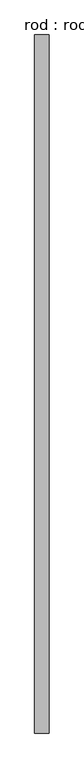
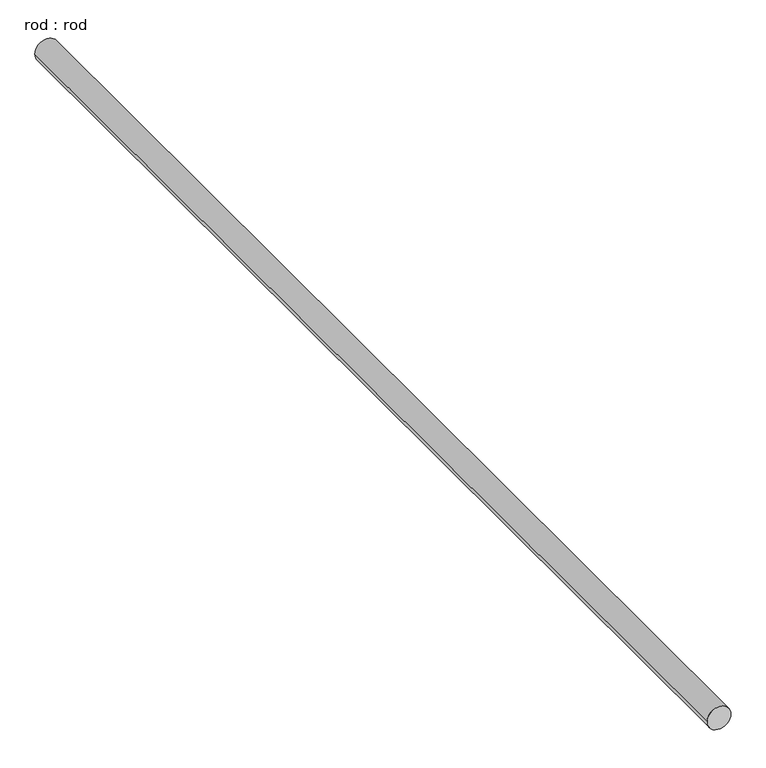
"""IFC4 building model written with IfcOpenShell, lengths in millimetres: proxy geometry, rod : rod."""

import ifcopenshell
import ifcopenshell.guid

model = None  # the IFC model being written
_history = None  # IfcOwnerHistory: only IFC2X3 demands one
_inside = {}  # id of a spatial element -> (the spatial element, [elements in it])
_under = {}  # id of a project, library or spatial element -> (it, [spatial elements below it])
_declared = {}  # id of a project -> (the project, [libraries it declares])
_typed = {}  # id of a type object -> (the type object, [elements of that type])
_made_of = {}  # id of a material, layer set ... -> (it, [elements and type objects made of it])


def new_model(schema):
    """Start an empty IFC model of exactly this schema.

    Asked for "IFC4X3", IfcOpenShell would pick the latest addendum, in which some entities
    have other attributes; the version numbers below select the first issue.
    IFC2X3 requires an IfcOwnerHistory on every rooted entity: one is made here for all.
    """
    global model, _history
    if schema == "IFC4X3":
        model = ifcopenshell.file(schema_version=(4, 3, 0, 0))
    else:
        model = ifcopenshell.file(schema=schema)
    _inside.clear()
    _under.clear()
    _declared.clear()
    _typed.clear()
    _made_of.clear()
    _history = None
    if model.schema == "IFC2X3":
        org = make("IfcOrganization", Name="unknown")
        user = make(
            "IfcPersonAndOrganization",
            ThePerson=make("IfcPerson", FamilyName="unknown"),
            TheOrganization=org,
        )
        app = make(
            "IfcApplication",
            ApplicationDeveloper=org,
            Version="unknown",
            ApplicationFullName="unknown",
            ApplicationIdentifier="unknown",
        )
        _history = make(
            "IfcOwnerHistory",
            OwningUser=user,
            OwningApplication=app,
            ChangeAction="ADDED",
            CreationDate=0,
        )
    return model


def make(cls, **values):
    """One entity of the class cls with the attributes given. An attribute that is None is left unset."""
    return model.create_entity(
        cls, **{name: value for name, value in values.items() if value is not None}
    )


def rooted(cls, **values):
    """An entity with a GlobalId (a new one), such as an element, a storey or a relation."""
    return make(cls, GlobalId=ifcopenshell.guid.new(), OwnerHistory=_history, **values)


def si_unit(unit_type, name, prefix=None):
    """IfcSIUnit, for example si_unit("LENGTHUNIT", "METRE", prefix="MILLI")."""
    return make("IfcSIUnit", UnitType=unit_type, Prefix=prefix, Name=name)


def assignment(units):
    """IfcUnitAssignment: the units of a project."""
    return None if units is None else make("IfcUnitAssignment", Units=units)


def point(xyz):
    """IfcCartesianPoint."""
    return None if xyz is None else make("IfcCartesianPoint", Coordinates=xyz)


def direction(xyz):
    """IfcDirection."""
    return None if xyz is None else make("IfcDirection", DirectionRatios=xyz)


def frame(location, z_axis=None, x_axis=None):
    """IfcAxis2Placement3D, a coordinate frame: its origin and axes. An axis left out is left unset."""
    return make(
        "IfcAxis2Placement3D",
        Location=point(location),
        Axis=direction(z_axis),
        RefDirection=direction(x_axis),
    )


def frame_2d(location, x_axis=None):
    """IfcAxis2Placement2D, a coordinate frame in the plane: its origin and x axis."""
    return make(
        "IfcAxis2Placement2D", Location=point(location), RefDirection=direction(x_axis)
    )


def origin():
    """The frame at (0, 0, 0) with its axes left unset."""
    return frame((0.0, 0.0, 0.0))


def place(relative_to, where):
    """IfcLocalPlacement: puts the frame where relative to a parent placement (None: the world)."""
    return make(
        "IfcLocalPlacement", PlacementRelTo=relative_to, RelativePlacement=where
    )


def context(
    kind, dimensions, precision=None, world=None, true_north=None, identifier=None
):
    """IfcGeometricRepresentationContext, for example the 3D "Model" context."""
    return make(
        "IfcGeometricRepresentationContext",
        ContextIdentifier=identifier,
        ContextType=kind,
        CoordinateSpaceDimension=dimensions,
        Precision=precision,
        WorldCoordinateSystem=world,
        TrueNorth=true_north,
    )


def project(units=None, contexts=None):
    """IfcProject with its units and contexts."""
    return rooted(
        "IfcProject",
        Name="project",
        RepresentationContexts=contexts,
        UnitsInContext=assignment(units),
    )


def spatial(cls, under=None, at=None, **own):
    """A site, building, storey or space (cls), placed at a placement, below another one or the project."""
    s = rooted(cls, ObjectPlacement=at, **own)
    if under is not None:
        _under.setdefault(under.id(), (under, []))[1].append(s)
    return s


def circle_curve(where, radius):
    """IfcCircle in the frame where."""
    return make("IfcCircle", Position=where, Radius=radius)


def trimmed(basis, trim1, trim2, sense, master):
    """IfcTrimmedCurve: the piece of a basis curve between two trims."""
    return make(
        "IfcTrimmedCurve",
        BasisCurve=basis,
        Trim1=trim1,
        Trim2=trim2,
        SenseAgreement=sense,
        MasterRepresentation=master,
    )


def segment(curve, same_sense, transition):
    """IfcCompositeCurveSegment."""
    return make(
        "IfcCompositeCurveSegment",
        Transition=transition,
        SameSense=same_sense,
        ParentCurve=curve,
    )


def composite_curve(segments, self_intersect=None):
    """IfcCompositeCurve: segments joined end to end."""
    return make("IfcCompositeCurve", Segments=segments, SelfIntersect=self_intersect)


def outline(outer, holes=None, kind="AREA"):
    """IfcArbitraryClosedProfileDef: a profile drawn as a closed curve; with holes, ...WithVoids."""
    if holes is None:
        return make("IfcArbitraryClosedProfileDef", ProfileType=kind, OuterCurve=outer)
    return make(
        "IfcArbitraryProfileDefWithVoids",
        ProfileType=kind,
        OuterCurve=outer,
        InnerCurves=holes,
    )


def extrude(swept, where, along, depth):
    """IfcExtrudedAreaSolid: the profile swept, set in the frame where, extruded along a direction by depth."""
    return make(
        "IfcExtrudedAreaSolid",
        SweptArea=swept,
        Position=where,
        ExtrudedDirection=direction(along),
        Depth=depth,
    )


def shape(context_of_items, identifier, shape_type, items):
    """IfcShapeRepresentation: the items that make up one representation, for example the "Body"."""
    return make(
        "IfcShapeRepresentation",
        ContextOfItems=context_of_items,
        RepresentationIdentifier=identifier,
        RepresentationType=shape_type,
        Items=items,
    )


def source(mapping_origin, context_of_items, identifier, shape_type, items):
    """IfcRepresentationMap: a shape defined once, which mapped items show again and again."""
    return make(
        "IfcRepresentationMap",
        MappingOrigin=mapping_origin,
        MappedRepresentation=shape(context_of_items, identifier, shape_type, items),
    )


def transform(
    local_origin,
    x_axis=None,
    y_axis=None,
    z_axis=None,
    scale=None,
    scale2=None,
    scale3=None,
    uniform=True,
):
    """IfcCartesianTransformationOperator3D, or its non-uniform kind. x_axis, y_axis, z_axis: its Axis1, 2, 3."""
    if uniform:
        return make(
            "IfcCartesianTransformationOperator3D",
            Axis1=direction(x_axis),
            Axis2=direction(y_axis),
            LocalOrigin=point(local_origin),
            Scale=scale,
            Axis3=direction(z_axis),
        )
    return make(
        "IfcCartesianTransformationOperator3DnonUniform",
        Axis1=direction(x_axis),
        Axis2=direction(y_axis),
        LocalOrigin=point(local_origin),
        Scale=scale,
        Axis3=direction(z_axis),
        Scale2=scale2,
        Scale3=scale3,
    )


def mapped(mapping_source, mapping_target):
    """IfcMappedItem: shows the shape of a source again, moved by a transform."""
    return make(
        "IfcMappedItem", MappingSource=mapping_source, MappingTarget=mapping_target
    )


def made_of(thing, what):
    """Note that an element or type object is made of a material, layer set ...; save() writes the relation."""
    if what is not None:
        _made_of.setdefault(what.id(), (what, []))[1].append(thing)
    return thing


def element(
    cls,
    number,
    at=None,
    inside=None,
    cuts=None,
    type_object=None,
    material=None,
    context=None,
    identifier="Body",
    shape_type=None,
    held_by="IfcProductDefinitionShape",
    body=None,
    shapes=None,
    **own,
):
    """One element of the class cls, such as IfcWall. Its Tag is "e" and its number.

    at: its placement. inside: the storey or other place that contains it. cuts: it is an
    opening in that element (IfcRelVoidsElement). A single representation is given by context,
    identifier, shape_type and body (its items); several are given by shapes. held_by: the class
    of the entity that holds the representations. save() writes the other relations.
    """
    e = rooted(cls, Tag="e%d" % number, ObjectPlacement=at, **own)
    if body is not None:
        shapes = [shape(context, identifier, shape_type, body)]
    if shapes is not None:
        e.Representation = make(held_by, Representations=shapes)
    if inside is not None:
        _inside.setdefault(inside.id(), (inside, []))[1].append(e)
    if cuts is not None:
        rooted(
            "IfcRelVoidsElement", RelatingBuildingElement=cuts, RelatedOpeningElement=e
        )
    if type_object is not None:
        _typed.setdefault(type_object.id(), (type_object, []))[1].append(e)
    return made_of(e, material)


def aggregate(whole, parts):
    """IfcRelAggregates: a whole, such as a stair, and the parts it consists of."""
    return rooted("IfcRelAggregates", RelatingObject=whole, RelatedObjects=parts)


def save(model, path):
    """Write the relations noted so far, then the file.

    IfcRelAggregates (storeys below a building ...), IfcRelContainedInSpatialStructure (elements
    in a storey), IfcRelDefinesByType, IfcRelAssociatesMaterial and IfcRelDeclares: one each for
    every whole, place, type object, material and project.
    """
    for whole, parts in _under.values():
        aggregate(whole, parts)
    for where, things in _inside.values():
        rooted(
            "IfcRelContainedInSpatialStructure",
            RelatedElements=things,
            RelatingStructure=where,
        )
    for kind, things in _typed.values():
        rooted("IfcRelDefinesByType", RelatedObjects=things, RelatingType=kind)
    for what, things in _made_of.values():
        rooted("IfcRelAssociatesMaterial", RelatedObjects=things, RelatingMaterial=what)
    for by, libraries in _declared.values():
        rooted("IfcRelDeclares", RelatingContext=by, RelatedDefinitions=libraries)
    model.write(path)


def rod_rod_b590edbd(model_context):
    return source(origin(), model_context, "Body", "SweptSolid", [
        extrude(outline(composite_curve([segment(trimmed(circle_curve(frame_2d((0.0108462, 0.0)), 200.0), [point((0.0108462, 200.0))], [point((0.0108462, -200.0))], False, "CARTESIAN"), True, "CONTINUOUS"), segment(trimmed(circle_curve(frame_2d((0.0108462, 0.0)), 200.0), [point((0.0108462, -200.0))], [point((0.0108462, 200.0))], False, "CARTESIAN"), True, "CONTINUOUS")], self_intersect=False)), frame((0.0, -5670.6642418, 0.0), z_axis=(0.0, 1.0, 0.0), x_axis=(0.0, 0.0, 1.0)), (0.0, 0.0, 1.0), 19526.7857143),
    ])


if __name__ == "__main__":
    model = new_model("IFC4")
    model_context = context("Model", 3, world=origin())
    ifc_project = project(units=[si_unit("LENGTHUNIT", "METRE", prefix="MILLI")], contexts=[model_context])
    site = spatial("IfcSite", under=ifc_project)
    building = spatial("IfcBuilding", under=site)
    placement = place(None, origin())
    rod_rod_shape = rod_rod_b590edbd(model_context)
    element("IfcBuildingElementProxy", 1, Name="rod : rod", ObjectType="rod : rod", at=placement, inside=building, context=model_context, shape_type="MappedRepresentation", body=[
        mapped(rod_rod_shape, transform((0.0, 0.0, 0.0), x_axis=(1.0, 0.0, 0.0), y_axis=(0.0, 1.0, 0.0), z_axis=(0.0, 0.0, 1.0))),
    ])
    save(model, "model.ifc")

# Revit data of these elements
# Type "rod : rod"
#   Default Elevation = 0
